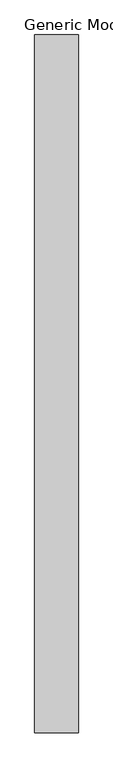
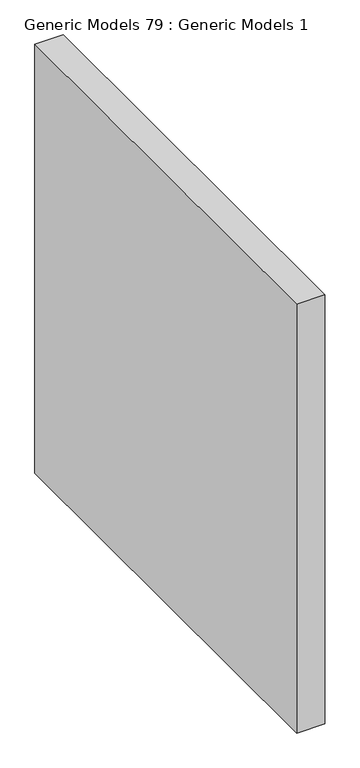
"""IFC4 building model written with IfcOpenShell, lengths in millimetres: proxy geometry, Generic Models 79 : Generic Models 1."""

import ifcopenshell
import ifcopenshell.guid

model = None  # the IFC model being written
_history = None  # IfcOwnerHistory: only IFC2X3 demands one
_inside = {}  # id of a spatial element -> (the spatial element, [elements in it])
_under = {}  # id of a project, library or spatial element -> (it, [spatial elements below it])
_declared = {}  # id of a project -> (the project, [libraries it declares])
_typed = {}  # id of a type object -> (the type object, [elements of that type])
_made_of = {}  # id of a material, layer set ... -> (it, [elements and type objects made of it])


def new_model(schema):
    """Start an empty IFC model of exactly this schema.

    Asked for "IFC4X3", IfcOpenShell would pick the latest addendum, in which some entities
    have other attributes; the version numbers below select the first issue.
    IFC2X3 requires an IfcOwnerHistory on every rooted entity: one is made here for all.
    """
    global model, _history
    if schema == "IFC4X3":
        model = ifcopenshell.file(schema_version=(4, 3, 0, 0))
    else:
        model = ifcopenshell.file(schema=schema)
    _inside.clear()
    _under.clear()
    _declared.clear()
    _typed.clear()
    _made_of.clear()
    _history = None
    if model.schema == "IFC2X3":
        org = make("IfcOrganization", Name="unknown")
        user = make(
            "IfcPersonAndOrganization",
            ThePerson=make("IfcPerson", FamilyName="unknown"),
            TheOrganization=org,
        )
        app = make(
            "IfcApplication",
            ApplicationDeveloper=org,
            Version="unknown",
            ApplicationFullName="unknown",
            ApplicationIdentifier="unknown",
        )
        _history = make(
            "IfcOwnerHistory",
            OwningUser=user,
            OwningApplication=app,
            ChangeAction="ADDED",
            CreationDate=0,
        )
    return model


def make(cls, **values):
    """One entity of the class cls with the attributes given. An attribute that is None is left unset."""
    return model.create_entity(
        cls, **{name: value for name, value in values.items() if value is not None}
    )


def rooted(cls, **values):
    """An entity with a GlobalId (a new one), such as an element, a storey or a relation."""
    return make(cls, GlobalId=ifcopenshell.guid.new(), OwnerHistory=_history, **values)


def si_unit(unit_type, name, prefix=None):
    """IfcSIUnit, for example si_unit("LENGTHUNIT", "METRE", prefix="MILLI")."""
    return make("IfcSIUnit", UnitType=unit_type, Prefix=prefix, Name=name)


def assignment(units):
    """IfcUnitAssignment: the units of a project."""
    return None if units is None else make("IfcUnitAssignment", Units=units)


def point(xyz):
    """IfcCartesianPoint."""
    return None if xyz is None else make("IfcCartesianPoint", Coordinates=xyz)


def direction(xyz):
    """IfcDirection."""
    return None if xyz is None else make("IfcDirection", DirectionRatios=xyz)


def frame(location, z_axis=None, x_axis=None):
    """IfcAxis2Placement3D, a coordinate frame: its origin and axes. An axis left out is left unset."""
    return make(
        "IfcAxis2Placement3D",
        Location=point(location),
        Axis=direction(z_axis),
        RefDirection=direction(x_axis),
    )


def origin():
    """The frame at (0, 0, 0) with its axes left unset."""
    return frame((0.0, 0.0, 0.0))


def place(relative_to, where):
    """IfcLocalPlacement: puts the frame where relative to a parent placement (None: the world)."""
    return make(
        "IfcLocalPlacement", PlacementRelTo=relative_to, RelativePlacement=where
    )


def context(
    kind, dimensions, precision=None, world=None, true_north=None, identifier=None
):
    """IfcGeometricRepresentationContext, for example the 3D "Model" context."""
    return make(
        "IfcGeometricRepresentationContext",
        ContextIdentifier=identifier,
        ContextType=kind,
        CoordinateSpaceDimension=dimensions,
        Precision=precision,
        WorldCoordinateSystem=world,
        TrueNorth=true_north,
    )


def project(units=None, contexts=None):
    """IfcProject with its units and contexts."""
    return rooted(
        "IfcProject",
        Name="project",
        RepresentationContexts=contexts,
        UnitsInContext=assignment(units),
    )


def spatial(cls, under=None, at=None, **own):
    """A site, building, storey or space (cls), placed at a placement, below another one or the project."""
    s = rooted(cls, ObjectPlacement=at, **own)
    if under is not None:
        _under.setdefault(under.id(), (under, []))[1].append(s)
    return s


def polyline(points):
    """IfcPolyline through the points."""
    return make("IfcPolyline", Points=[point(p) for p in points])


def outline(outer, holes=None, kind="AREA"):
    """IfcArbitraryClosedProfileDef: a profile drawn as a closed curve; with holes, ...WithVoids."""
    if holes is None:
        return make("IfcArbitraryClosedProfileDef", ProfileType=kind, OuterCurve=outer)
    return make(
        "IfcArbitraryProfileDefWithVoids",
        ProfileType=kind,
        OuterCurve=outer,
        InnerCurves=holes,
    )


def extrude(swept, where, along, depth):
    """IfcExtrudedAreaSolid: the profile swept, set in the frame where, extruded along a direction by depth."""
    return make(
        "IfcExtrudedAreaSolid",
        SweptArea=swept,
        Position=where,
        ExtrudedDirection=direction(along),
        Depth=depth,
    )


def shape(context_of_items, identifier, shape_type, items):
    """IfcShapeRepresentation: the items that make up one representation, for example the "Body"."""
    return make(
        "IfcShapeRepresentation",
        ContextOfItems=context_of_items,
        RepresentationIdentifier=identifier,
        RepresentationType=shape_type,
        Items=items,
    )


def source(mapping_origin, context_of_items, identifier, shape_type, items):
    """IfcRepresentationMap: a shape defined once, which mapped items show again and again."""
    return make(
        "IfcRepresentationMap",
        MappingOrigin=mapping_origin,
        MappedRepresentation=shape(context_of_items, identifier, shape_type, items),
    )


def transform(
    local_origin,
    x_axis=None,
    y_axis=None,
    z_axis=None,
    scale=None,
    scale2=None,
    scale3=None,
    uniform=True,
):
    """IfcCartesianTransformationOperator3D, or its non-uniform kind. x_axis, y_axis, z_axis: its Axis1, 2, 3."""
    if uniform:
        return make(
            "IfcCartesianTransformationOperator3D",
            Axis1=direction(x_axis),
            Axis2=direction(y_axis),
            LocalOrigin=point(local_origin),
            Scale=scale,
            Axis3=direction(z_axis),
        )
    return make(
        "IfcCartesianTransformationOperator3DnonUniform",
        Axis1=direction(x_axis),
        Axis2=direction(y_axis),
        LocalOrigin=point(local_origin),
        Scale=scale,
        Axis3=direction(z_axis),
        Scale2=scale2,
        Scale3=scale3,
    )


def mapped(mapping_source, mapping_target):
    """IfcMappedItem: shows the shape of a source again, moved by a transform."""
    return make(
        "IfcMappedItem", MappingSource=mapping_source, MappingTarget=mapping_target
    )


def made_of(thing, what):
    """Note that an element or type object is made of a material, layer set ...; save() writes the relation."""
    if what is not None:
        _made_of.setdefault(what.id(), (what, []))[1].append(thing)
    return thing


def element(
    cls,
    number,
    at=None,
    inside=None,
    cuts=None,
    type_object=None,
    material=None,
    context=None,
    identifier="Body",
    shape_type=None,
    held_by="IfcProductDefinitionShape",
    body=None,
    shapes=None,
    **own,
):
    """One element of the class cls, such as IfcWall. Its Tag is "e" and its number.

    at: its placement. inside: the storey or other place that contains it. cuts: it is an
    opening in that element (IfcRelVoidsElement). A single representation is given by context,
    identifier, shape_type and body (its items); several are given by shapes. held_by: the class
    of the entity that holds the representations. save() writes the other relations.
    """
    e = rooted(cls, Tag="e%d" % number, ObjectPlacement=at, **own)
    if body is not None:
        shapes = [shape(context, identifier, shape_type, body)]
    if shapes is not None:
        e.Representation = make(held_by, Representations=shapes)
    if inside is not None:
        _inside.setdefault(inside.id(), (inside, []))[1].append(e)
    if cuts is not None:
        rooted(
            "IfcRelVoidsElement", RelatingBuildingElement=cuts, RelatedOpeningElement=e
        )
    if type_object is not None:
        _typed.setdefault(type_object.id(), (type_object, []))[1].append(e)
    return made_of(e, material)


def aggregate(whole, parts):
    """IfcRelAggregates: a whole, such as a stair, and the parts it consists of."""
    return rooted("IfcRelAggregates", RelatingObject=whole, RelatedObjects=parts)


def save(model, path):
    """Write the relations noted so far, then the file.

    IfcRelAggregates (storeys below a building ...), IfcRelContainedInSpatialStructure (elements
    in a storey), IfcRelDefinesByType, IfcRelAssociatesMaterial and IfcRelDeclares: one each for
    every whole, place, type object, material and project.
    """
    for whole, parts in _under.values():
        aggregate(whole, parts)
    for where, things in _inside.values():
        rooted(
            "IfcRelContainedInSpatialStructure",
            RelatedElements=things,
            RelatingStructure=where,
        )
    for kind, things in _typed.values():
        rooted("IfcRelDefinesByType", RelatedObjects=things, RelatingType=kind)
    for what, things in _made_of.values():
        rooted("IfcRelAssociatesMaterial", RelatedObjects=things, RelatingMaterial=what)
    for by, libraries in _declared.values():
        rooted("IfcRelDeclares", RelatingContext=by, RelatedDefinitions=libraries)
    model.write(path)


def generic_models_79_generic_models_1_6d14886f(model_context):
    return source(origin(), model_context, "Body", "SweptSolid", [
        extrude(outline(polyline([(49776.0625, 0.0), (49699.8625, 0.0), (49699.8625, 1219.2), (49776.0625, 1219.2), (49776.0625, 0.0)])), frame((0.0, 0.0, 29.437912), z_axis=(0.0, 0.0, 1.0), x_axis=(1.0, 0.0, 0.0)), (0.0, 0.0, 1.0), 1219.2),
    ])


if __name__ == "__main__":
    model = new_model("IFC4")
    model_context = context("Model", 3, world=origin())
    ifc_project = project(units=[si_unit("LENGTHUNIT", "METRE", prefix="MILLI")], contexts=[model_context])
    site = spatial("IfcSite", under=ifc_project)
    building = spatial("IfcBuilding", under=site)
    placement = place(None, origin())
    generic_models_79_generic_models_1_shape = generic_models_79_generic_models_1_6d14886f(model_context)
    element("IfcBuildingElementProxy", 1, Name="Generic Models 79 : Generic Models 1", ObjectType="Generic Models 79 : Generic Models 1", at=placement, inside=building, context=model_context, shape_type="MappedRepresentation", body=[
        mapped(generic_models_79_generic_models_1_shape, transform((0.0, 0.0, 0.0), x_axis=(1.0, 0.0, 0.0), y_axis=(0.0, 1.0, 0.0), z_axis=(0.0, 0.0, 1.0))),
    ])
    save(model, "model.ifc")

# Revit data of these elements
# Element 1 (IfcBuildingElementProxy, "Generic Models 79 : Generic Models 1")
#   Materials on its faces: "SOUND BATT. INSULATION (THICKNESS TO MATCH WALL DEPTH)"
# Materials
#   "SOUND BATT. INSULATION (THICKNESS TO MATCH WALL DEPTH)": class "Unassigned", colour RGB 255 255 255, transparency 0, Cost = 0
